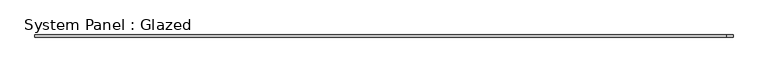
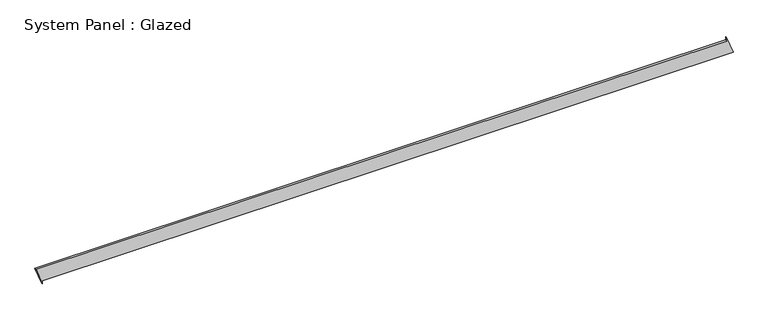
"""IFC4 building model written with IfcOpenShell, lengths in millimetres: plate geometry, System Panel : Glazed."""

from ifc_helpers import new_model, si_unit, frame, origin, place, context, project, spatial, polyline, outline, extrude, source, transform, mapped, element, save


def system_panel_glazed_2fdd73bd(model_context):
    return source(origin(), model_context, "Body", "SweptSolid", [
        extrude(outline(polyline([(0.0, -3957.1351812), (35.3553391, -3957.1351812), (35.3553391, 4028.2169221), (234.3998836, 3956.3375389), (199.0445445, 3956.3360146), (199.3887904, -4028.2169221), (0.0, -3957.1351812)])), frame((0.0, -49.5, 0.0), z_axis=(0.0, 1.0, 0.0), x_axis=(0.0, 0.0, 1.0)), (0.0, 0.0, 1.0), 25.0),
    ])


if __name__ == "__main__":
    model = new_model("IFC4")
    model_context = context("Model", 3, world=origin())
    ifc_project = project(units=[si_unit("LENGTHUNIT", "METRE", prefix="MILLI")], contexts=[model_context])
    site = spatial("IfcSite", under=ifc_project)
    building = spatial("IfcBuilding", under=site)
    placement = place(None, origin())
    system_panel_glazed_shape = system_panel_glazed_2fdd73bd(model_context)
    element("IfcPlate", 1, ObjectType="System Panel : Glazed", at=placement, inside=building, context=model_context, shape_type="MappedRepresentation", body=[
        mapped(system_panel_glazed_shape, transform((0.0, 0.0, 0.0), x_axis=(1.0, 0.0, 0.0), y_axis=(0.0, 1.0, 0.0), z_axis=(0.0, 0.0, 1.0))),
    ])
    save(model, "model.ifc")

# Revit data of these elements
# Element 1 (IfcPlate, "System Panel : Glazed")
#   Materials on its faces: "Glass"
# Materials
#   "Glass": class "Glass", colour RGB 218 227 224, transparency 0.85, Description = "Soda Lime Glass", Cost = 0
